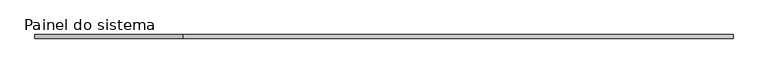
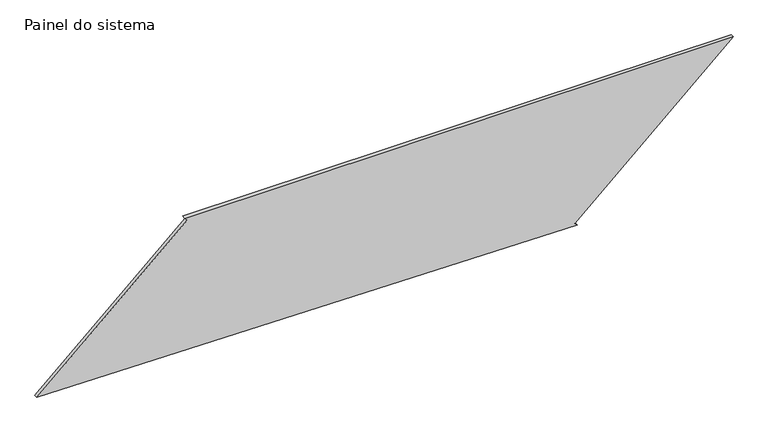
"""IFC4 building model written with IfcOpenShell, lengths in millimetres: plate geometry, Painel do sistema : Envidraçado."""

import ifcopenshell
import ifcopenshell.guid

model = None  # the IFC model being written
_history = None  # IfcOwnerHistory: only IFC2X3 demands one
_inside = {}  # id of a spatial element -> (the spatial element, [elements in it])
_under = {}  # id of a project, library or spatial element -> (it, [spatial elements below it])
_declared = {}  # id of a project -> (the project, [libraries it declares])
_typed = {}  # id of a type object -> (the type object, [elements of that type])
_made_of = {}  # id of a material, layer set ... -> (it, [elements and type objects made of it])


def new_model(schema):
    """Start an empty IFC model of exactly this schema.

    Asked for "IFC4X3", IfcOpenShell would pick the latest addendum, in which some entities
    have other attributes; the version numbers below select the first issue.
    IFC2X3 requires an IfcOwnerHistory on every rooted entity: one is made here for all.
    """
    global model, _history
    if schema == "IFC4X3":
        model = ifcopenshell.file(schema_version=(4, 3, 0, 0))
    else:
        model = ifcopenshell.file(schema=schema)
    _inside.clear()
    _under.clear()
    _declared.clear()
    _typed.clear()
    _made_of.clear()
    _history = None
    if model.schema == "IFC2X3":
        org = make("IfcOrganization", Name="unknown")
        user = make(
            "IfcPersonAndOrganization",
            ThePerson=make("IfcPerson", FamilyName="unknown"),
            TheOrganization=org,
        )
        app = make(
            "IfcApplication",
            ApplicationDeveloper=org,
            Version="unknown",
            ApplicationFullName="unknown",
            ApplicationIdentifier="unknown",
        )
        _history = make(
            "IfcOwnerHistory",
            OwningUser=user,
            OwningApplication=app,
            ChangeAction="ADDED",
            CreationDate=0,
        )
    return model


def make(cls, **values):
    """One entity of the class cls with the attributes given. An attribute that is None is left unset."""
    return model.create_entity(
        cls, **{name: value for name, value in values.items() if value is not None}
    )


def rooted(cls, **values):
    """An entity with a GlobalId (a new one), such as an element, a storey or a relation."""
    return make(cls, GlobalId=ifcopenshell.guid.new(), OwnerHistory=_history, **values)


def si_unit(unit_type, name, prefix=None):
    """IfcSIUnit, for example si_unit("LENGTHUNIT", "METRE", prefix="MILLI")."""
    return make("IfcSIUnit", UnitType=unit_type, Prefix=prefix, Name=name)


def assignment(units):
    """IfcUnitAssignment: the units of a project."""
    return None if units is None else make("IfcUnitAssignment", Units=units)


def point(xyz):
    """IfcCartesianPoint."""
    return None if xyz is None else make("IfcCartesianPoint", Coordinates=xyz)


def direction(xyz):
    """IfcDirection."""
    return None if xyz is None else make("IfcDirection", DirectionRatios=xyz)


def frame(location, z_axis=None, x_axis=None):
    """IfcAxis2Placement3D, a coordinate frame: its origin and axes. An axis left out is left unset."""
    return make(
        "IfcAxis2Placement3D",
        Location=point(location),
        Axis=direction(z_axis),
        RefDirection=direction(x_axis),
    )


def origin():
    """The frame at (0, 0, 0) with its axes left unset."""
    return frame((0.0, 0.0, 0.0))


def place(relative_to, where):
    """IfcLocalPlacement: puts the frame where relative to a parent placement (None: the world)."""
    return make(
        "IfcLocalPlacement", PlacementRelTo=relative_to, RelativePlacement=where
    )


def context(
    kind, dimensions, precision=None, world=None, true_north=None, identifier=None
):
    """IfcGeometricRepresentationContext, for example the 3D "Model" context."""
    return make(
        "IfcGeometricRepresentationContext",
        ContextIdentifier=identifier,
        ContextType=kind,
        CoordinateSpaceDimension=dimensions,
        Precision=precision,
        WorldCoordinateSystem=world,
        TrueNorth=true_north,
    )


def project(units=None, contexts=None):
    """IfcProject with its units and contexts."""
    return rooted(
        "IfcProject",
        Name="project",
        RepresentationContexts=contexts,
        UnitsInContext=assignment(units),
    )


def spatial(cls, under=None, at=None, **own):
    """A site, building, storey or space (cls), placed at a placement, below another one or the project."""
    s = rooted(cls, ObjectPlacement=at, **own)
    if under is not None:
        _under.setdefault(under.id(), (under, []))[1].append(s)
    return s


def polyline(points):
    """IfcPolyline through the points."""
    return make("IfcPolyline", Points=[point(p) for p in points])


def outline(outer, holes=None, kind="AREA"):
    """IfcArbitraryClosedProfileDef: a profile drawn as a closed curve; with holes, ...WithVoids."""
    if holes is None:
        return make("IfcArbitraryClosedProfileDef", ProfileType=kind, OuterCurve=outer)
    return make(
        "IfcArbitraryProfileDefWithVoids",
        ProfileType=kind,
        OuterCurve=outer,
        InnerCurves=holes,
    )


def extrude(swept, where, along, depth):
    """IfcExtrudedAreaSolid: the profile swept, set in the frame where, extruded along a direction by depth."""
    return make(
        "IfcExtrudedAreaSolid",
        SweptArea=swept,
        Position=where,
        ExtrudedDirection=direction(along),
        Depth=depth,
    )


def shape(context_of_items, identifier, shape_type, items):
    """IfcShapeRepresentation: the items that make up one representation, for example the "Body"."""
    return make(
        "IfcShapeRepresentation",
        ContextOfItems=context_of_items,
        RepresentationIdentifier=identifier,
        RepresentationType=shape_type,
        Items=items,
    )


def source(mapping_origin, context_of_items, identifier, shape_type, items):
    """IfcRepresentationMap: a shape defined once, which mapped items show again and again."""
    return make(
        "IfcRepresentationMap",
        MappingOrigin=mapping_origin,
        MappedRepresentation=shape(context_of_items, identifier, shape_type, items),
    )


def transform(
    local_origin,
    x_axis=None,
    y_axis=None,
    z_axis=None,
    scale=None,
    scale2=None,
    scale3=None,
    uniform=True,
):
    """IfcCartesianTransformationOperator3D, or its non-uniform kind. x_axis, y_axis, z_axis: its Axis1, 2, 3."""
    if uniform:
        return make(
            "IfcCartesianTransformationOperator3D",
            Axis1=direction(x_axis),
            Axis2=direction(y_axis),
            LocalOrigin=point(local_origin),
            Scale=scale,
            Axis3=direction(z_axis),
        )
    return make(
        "IfcCartesianTransformationOperator3DnonUniform",
        Axis1=direction(x_axis),
        Axis2=direction(y_axis),
        LocalOrigin=point(local_origin),
        Scale=scale,
        Axis3=direction(z_axis),
        Scale2=scale2,
        Scale3=scale3,
    )


def mapped(mapping_source, mapping_target):
    """IfcMappedItem: shows the shape of a source again, moved by a transform."""
    return make(
        "IfcMappedItem", MappingSource=mapping_source, MappingTarget=mapping_target
    )


def made_of(thing, what):
    """Note that an element or type object is made of a material, layer set ...; save() writes the relation."""
    if what is not None:
        _made_of.setdefault(what.id(), (what, []))[1].append(thing)
    return thing


def element(
    cls,
    number,
    at=None,
    inside=None,
    cuts=None,
    type_object=None,
    material=None,
    context=None,
    identifier="Body",
    shape_type=None,
    held_by="IfcProductDefinitionShape",
    body=None,
    shapes=None,
    **own,
):
    """One element of the class cls, such as IfcWall. Its Tag is "e" and its number.

    at: its placement. inside: the storey or other place that contains it. cuts: it is an
    opening in that element (IfcRelVoidsElement). A single representation is given by context,
    identifier, shape_type and body (its items); several are given by shapes. held_by: the class
    of the entity that holds the representations. save() writes the other relations.
    """
    e = rooted(cls, Tag="e%d" % number, ObjectPlacement=at, **own)
    if body is not None:
        shapes = [shape(context, identifier, shape_type, body)]
    if shapes is not None:
        e.Representation = make(held_by, Representations=shapes)
    if inside is not None:
        _inside.setdefault(inside.id(), (inside, []))[1].append(e)
    if cuts is not None:
        rooted(
            "IfcRelVoidsElement", RelatingBuildingElement=cuts, RelatedOpeningElement=e
        )
    if type_object is not None:
        _typed.setdefault(type_object.id(), (type_object, []))[1].append(e)
    return made_of(e, material)


def aggregate(whole, parts):
    """IfcRelAggregates: a whole, such as a stair, and the parts it consists of."""
    return rooted("IfcRelAggregates", RelatingObject=whole, RelatedObjects=parts)


def save(model, path):
    """Write the relations noted so far, then the file.

    IfcRelAggregates (storeys below a building ...), IfcRelContainedInSpatialStructure (elements
    in a storey), IfcRelDefinesByType, IfcRelAssociatesMaterial and IfcRelDeclares: one each for
    every whole, place, type object, material and project.
    """
    for whole, parts in _under.values():
        aggregate(whole, parts)
    for where, things in _inside.values():
        rooted(
            "IfcRelContainedInSpatialStructure",
            RelatedElements=things,
            RelatingStructure=where,
        )
    for kind, things in _typed.values():
        rooted("IfcRelDefinesByType", RelatedObjects=things, RelatingType=kind)
    for what, things in _made_of.values():
        rooted("IfcRelAssociatesMaterial", RelatedObjects=things, RelatingMaterial=what)
    for by, libraries in _declared.values():
        rooted("IfcRelDeclares", RelatingContext=by, RelatedDefinitions=libraries)
    model.write(path)


def painel_do_sistema_ea64a829(model_context):
    return source(origin(), model_context, "Body", "SweptSolid", [
        extrude(outline(polyline([(0.0, 1337.0716199), (18.5968466, 1320.363619), (1006.6876924, 2420.1585009), (1006.6876924, -1391.830958), (988.0908458, -1375.1229571), (49.1975382, -2420.1585009), (0.0, 1337.0716199)])), frame((0.0, 24.5, 0.0), z_axis=(0.0, 1.0, 0.0), x_axis=(0.0, 0.0, 1.0)), (0.0, 0.0, 1.0), 25.0),
    ])


if __name__ == "__main__":
    model = new_model("IFC4")
    model_context = context("Model", 3, world=origin())
    ifc_project = project(units=[si_unit("LENGTHUNIT", "METRE", prefix="MILLI")], contexts=[model_context])
    site = spatial("IfcSite", under=ifc_project)
    building = spatial("IfcBuilding", under=site)
    placement = place(None, origin())
    painel_do_sistema_shape = painel_do_sistema_ea64a829(model_context)
    element("IfcPlate", 1, ObjectType="Painel do sistema : Envidraçado", at=placement, inside=building, context=model_context, shape_type="MappedRepresentation", body=[
        mapped(painel_do_sistema_shape, transform((0.0, 0.0, 0.0), x_axis=(1.0, 0.0, 0.0), y_axis=(0.0, 1.0, 0.0), z_axis=(0.0, 0.0, 1.0))),
    ])
    save(model, "model.ifc")

# Revit data of these elements
# Type "Painel do sistema : Envidraçado"
#   Construction Type Id = "GSP4R"
#   Analytic Construction = "Vidraça única Pilkington 1/8 pol"
#   Visual Light Transmittance = 0.9
#   Solar Heat Gain Coefficient = 0.86
#   Heat Transfer Coefficient (U) = 6.7069 W/(m²·K)
# Element 1 (IfcPlate, "Painel do sistema : Envidraçado")
#   Materials on its faces: "Vidro"
# Materials
#   "Vidro": class "Vidro", colour RGB 0 128 192, transparency 0.9, Description = "Vidro de sílica", Cost = 0
